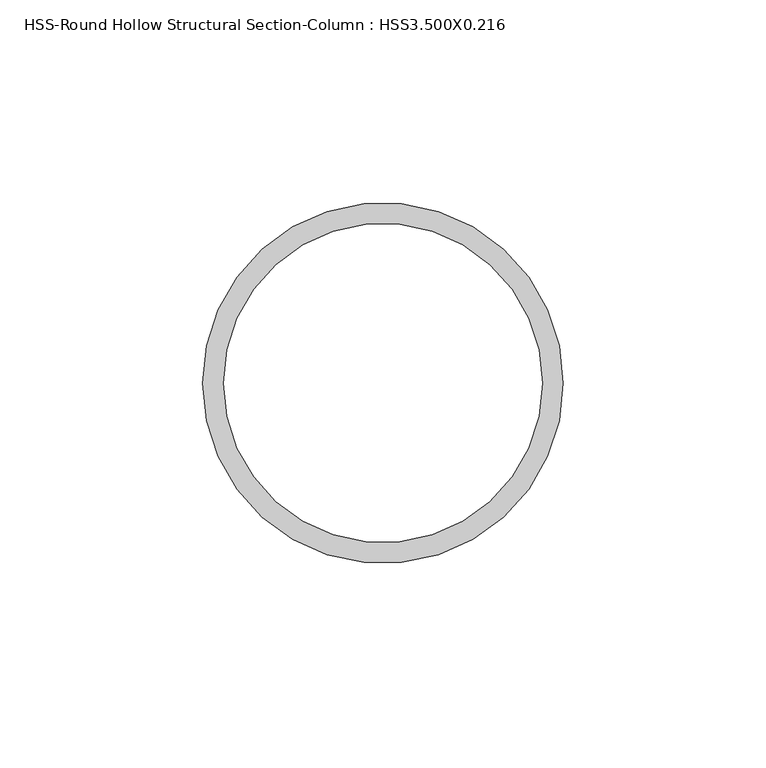
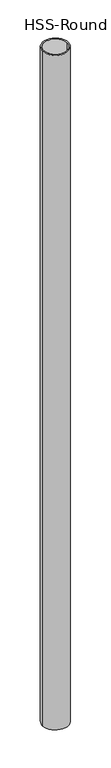
"""IFC4 building model written with IfcOpenShell, lengths in millimetres: column geometry, HSS-Round Hollow Structural Section-Column : HSS3.500X0.216."""

from ifc_helpers import new_model, si_unit, point, frame, origin, origin_2d, place, context, project, spatial, circle_curve, trimmed, segment, composite_curve, outline, extrude, source, transform, mapped, element, save


def hss_round_hollow_structural_section_column_hss3_500x0_216_7bbf5c96(model_context):
    return source(origin(), model_context, "Body", "SweptSolid", [
        extrude(outline(composite_curve([segment(trimmed(circle_curve(origin_2d(), 44.45), [point((-44.45, 0.0))], [point((44.45, 0.0))], False, "CARTESIAN"), True, "CONTINUOUS"), segment(trimmed(circle_curve(origin_2d(), 44.45), [point((44.45, 0.0))], [point((-44.45, 0.0))], False, "CARTESIAN"), True, "CONTINUOUS")], self_intersect=False), holes=[composite_curve([segment(trimmed(circle_curve(origin_2d(), 39.3446), [point((-39.3446, 0.0))], [point((39.3446, 0.0))], True, "CARTESIAN"), True, "CONTINUOUS"), segment(trimmed(circle_curve(origin_2d(), 39.3446), [point((39.3446, 0.0))], [point((-39.3446, 0.0))], True, "CARTESIAN"), True, "CONTINUOUS")], self_intersect=False)]), frame((0.0, 0.0, -2438.4), z_axis=(0.0, 0.0, 1.0), x_axis=(1.0, 0.0, 0.0)), (0.0, 0.0, 1.0), 2438.4),
    ])


if __name__ == "__main__":
    model = new_model("IFC4")
    model_context = context("Model", 3, world=origin())
    ifc_project = project(units=[si_unit("LENGTHUNIT", "METRE", prefix="MILLI")], contexts=[model_context])
    site = spatial("IfcSite", under=ifc_project)
    building = spatial("IfcBuilding", under=site)
    placement = place(None, origin())
    hss_round_hollow_structural_section_column_hss3_500x0_216_shape = hss_round_hollow_structural_section_column_hss3_500x0_216_7bbf5c96(model_context)
    element("IfcColumn", 1, ObjectType="HSS-Round Hollow Structural Section-Column : HSS3.500X0.216", at=placement, inside=building, context=model_context, shape_type="MappedRepresentation", body=[
        mapped(hss_round_hollow_structural_section_column_hss3_500x0_216_shape, transform((0.0, 0.0, 0.0), x_axis=(1.0, 0.0, 0.0), y_axis=(0.0, 1.0, 0.0), z_axis=(0.0, 0.0, 1.0))),
    ])
    save(model, "model.ifc")

# Revit data of these elements
# Type "HSS-Round Hollow Structural Section-Column : HSS3.500X0.216"
#   Assembly Code = "B10"
#   W = 7.58
#   OD = 0' - 3 1/2"
#   t = 0' - 0.201"
#   A = 0.0144444 SF
#   Structural Material [instance default] = Steel ASTM A53
# Element 1 (IfcColumn, "HSS-Round Hollow Structural Section-Column : HSS3.500X0.216")
#   Materials on its faces: "Steel ASTM A53"
# Materials
#   "Steel ASTM A53": class "Metal", colour RGB 199 199 199, transparency 0, Description = "Carbon steel", Cost = 0
